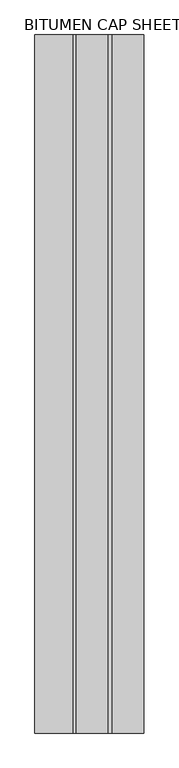
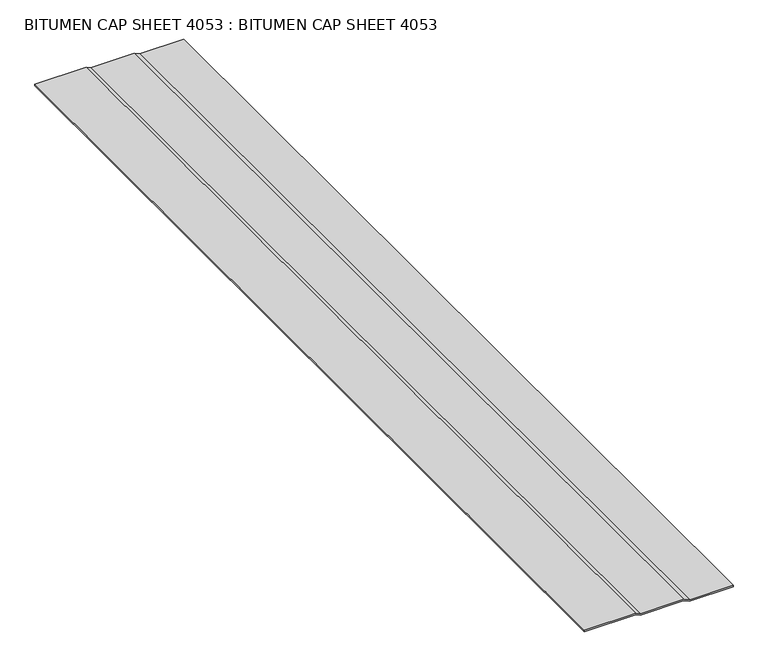
"""IFC4 building model written with IfcOpenShell, lengths in millimetres: proxy geometry, BITUMEN CAP SHEET 4053 : BITUMEN CAP SHEET 4053."""

from ifc_helpers import new_model, si_unit, frame, origin, place, context, project, spatial, polyline, outline, extrude, source, transform, mapped, element, save


def bitumen_cap_sheet_4053_bitumen_cap_sheet_4053_313e2dc3(model_context):
    return source(origin(), model_context, "Body", "SweptSolid", [
        extrude(outline(polyline([(40259.2002678, -2469.2761954), (40262.3752678, -2469.2761954), (40262.3752678, -2560.795457), (40267.6612773, -2573.2602756), (40267.6612773, -2663.9440313), (40271.9940719, -2673.6609328), (40271.9940719, -2781.5474293), (40268.8188423, -2781.5474293), (40268.8188423, -2674.3362183), (40264.4862773, -2664.6198318), (40264.4862773, -2573.9056756), (40259.2002678, -2561.440857), (40259.2002678, -2469.2761954)])), frame((0.0, -1052.8906574, 0.0), z_axis=(0.0, 1.0, 0.0), x_axis=(0.0, 0.0, 1.0)), (0.0, 0.0, 1.0), 2000.25),
    ])


if __name__ == "__main__":
    model = new_model("IFC4")
    model_context = context("Model", 3, world=origin())
    ifc_project = project(units=[si_unit("LENGTHUNIT", "METRE", prefix="MILLI")], contexts=[model_context])
    site = spatial("IfcSite", under=ifc_project)
    building = spatial("IfcBuilding", under=site)
    placement = place(None, origin())
    bitumen_cap_sheet_4053_bitumen_cap_sheet_4053_shape = bitumen_cap_sheet_4053_bitumen_cap_sheet_4053_313e2dc3(model_context)
    element("IfcBuildingElementProxy", 1, Name="BITUMEN CAP SHEET 4053 : BITUMEN CAP SHEET 4053", ObjectType="BITUMEN CAP SHEET 4053 : BITUMEN CAP SHEET 4053", at=placement, inside=building, context=model_context, shape_type="MappedRepresentation", body=[
        mapped(bitumen_cap_sheet_4053_bitumen_cap_sheet_4053_shape, transform((0.0, 0.0, 0.0), x_axis=(1.0, 0.0, 0.0), y_axis=(0.0, 1.0, 0.0), z_axis=(0.0, 0.0, 1.0))),
    ])
    save(model, "model.ifc")

# Revit data of these elements
# Type "BITUMEN CAP SHEET 4053 : BITUMEN CAP SHEET 4053"
#   NameOverride = "BITUMEN CAP SHEET"
# Element 1 (IfcBuildingElementProxy, "BITUMEN CAP SHEET 4053 : BITUMEN CAP SHEET 4053")
#   Materials on its faces: "MODIFIED BITUMEN GRANULE SURFACED CAP SHEET"
# Materials
#   "MODIFIED BITUMEN GRANULE SURFACED CAP SHEET": class "Unassigned", colour RGB 85 85 127, transparency 0
